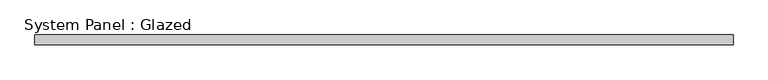
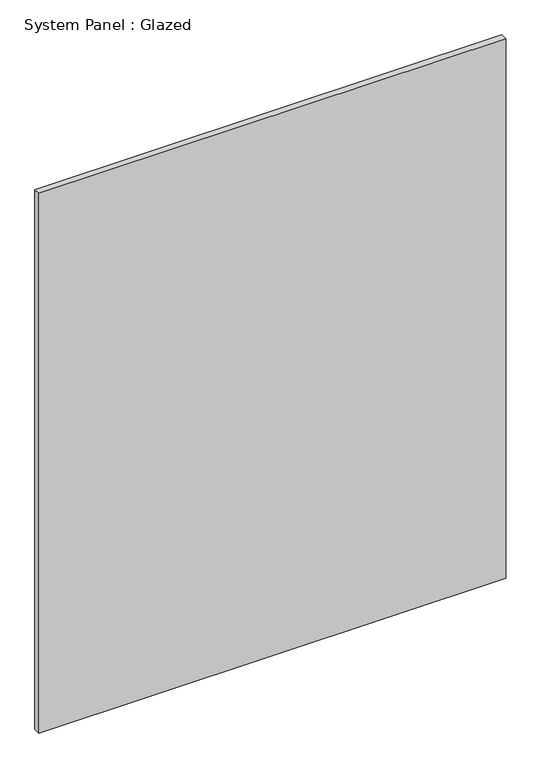
"""IFC4 building model written with IfcOpenShell, lengths in millimetres: plate geometry, System Panel : Glazed."""

from ifc_helpers import new_model, si_unit, origin, origin_with_axes, place, context, project, spatial, polyline, outline, extrude, source, transform, mapped, element, save


def system_panel_glazed_f186845e(model_context):
    return source(origin(), model_context, "Body", "SweptSolid", [
        extrude(outline(polyline([(879.5, -49.5), (-879.5, -49.5), (-879.5, -24.5), (879.5, -24.5), (879.5, -49.5)])), origin_with_axes(), (0.0, 0.0, 1.0), 2150.0),
    ])


if __name__ == "__main__":
    model = new_model("IFC4")
    model_context = context("Model", 3, world=origin())
    ifc_project = project(units=[si_unit("LENGTHUNIT", "METRE", prefix="MILLI")], contexts=[model_context])
    site = spatial("IfcSite", under=ifc_project)
    building = spatial("IfcBuilding", under=site)
    placement = place(None, origin())
    system_panel_glazed_shape = system_panel_glazed_f186845e(model_context)
    element("IfcPlate", 1, ObjectType="System Panel : Glazed", at=placement, inside=building, context=model_context, shape_type="MappedRepresentation", body=[
        mapped(system_panel_glazed_shape, transform((0.0, 0.0, 0.0), x_axis=(1.0, 0.0, 0.0), y_axis=(0.0, 1.0, 0.0), z_axis=(0.0, 0.0, 1.0))),
    ])
    save(model, "model.ifc")

# Revit data of these elements
# Type "System Panel : Glazed"
#   Keynote = "H11"
#   Construction Type Id = "GSP4R"
#   Analytic Construction = "1/8 in Pilkington single glazing"
#   Visual Light Transmittance = 0.9
#   Solar Heat Gain Coefficient = 0.86
#   Heat Transfer Coefficient (U) = 6.7069 W/(m²·K)
# Element 1 (IfcPlate, "System Panel : Glazed")
#   Materials on its faces: "Glass"
# Materials
#   "Glass": class "Glass", colour RGB 0 128 192, transparency 0.9, Description = "Soda Lime Glass", Cost = 0
